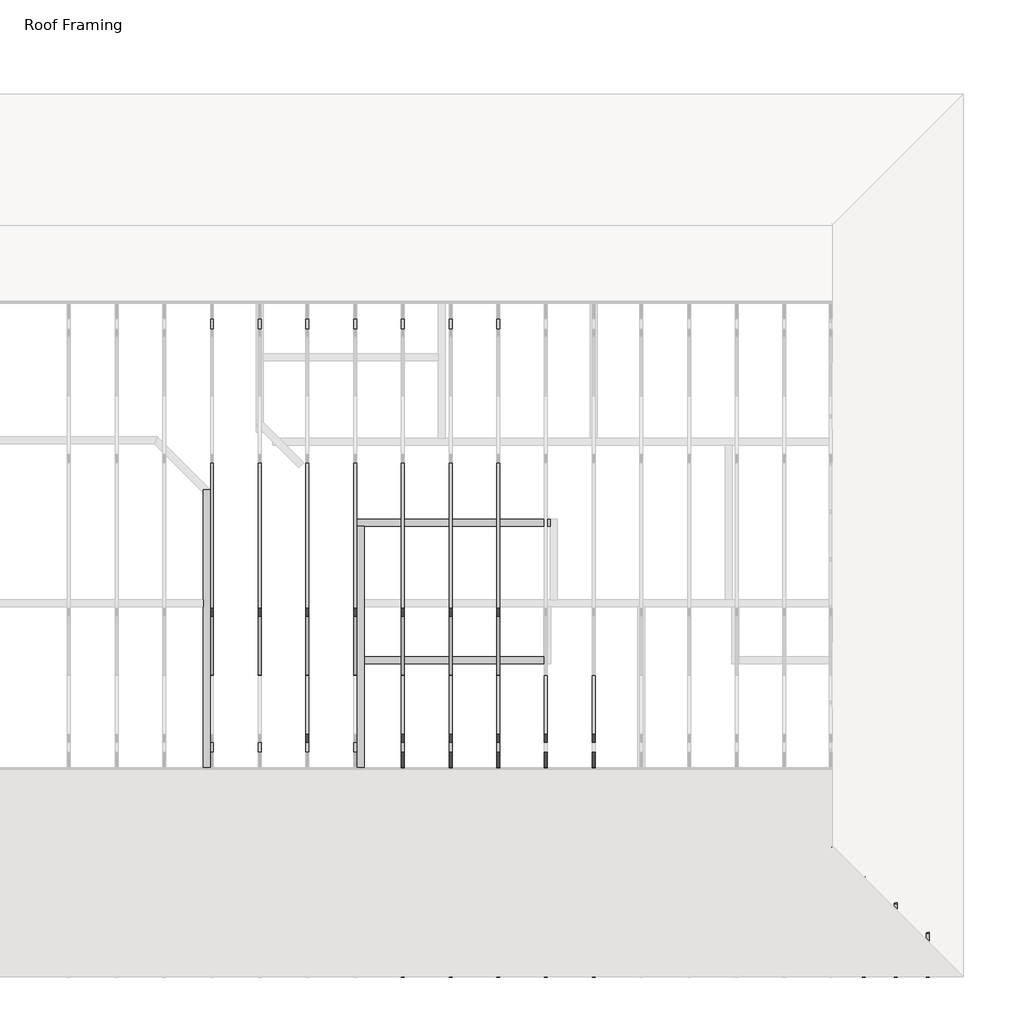
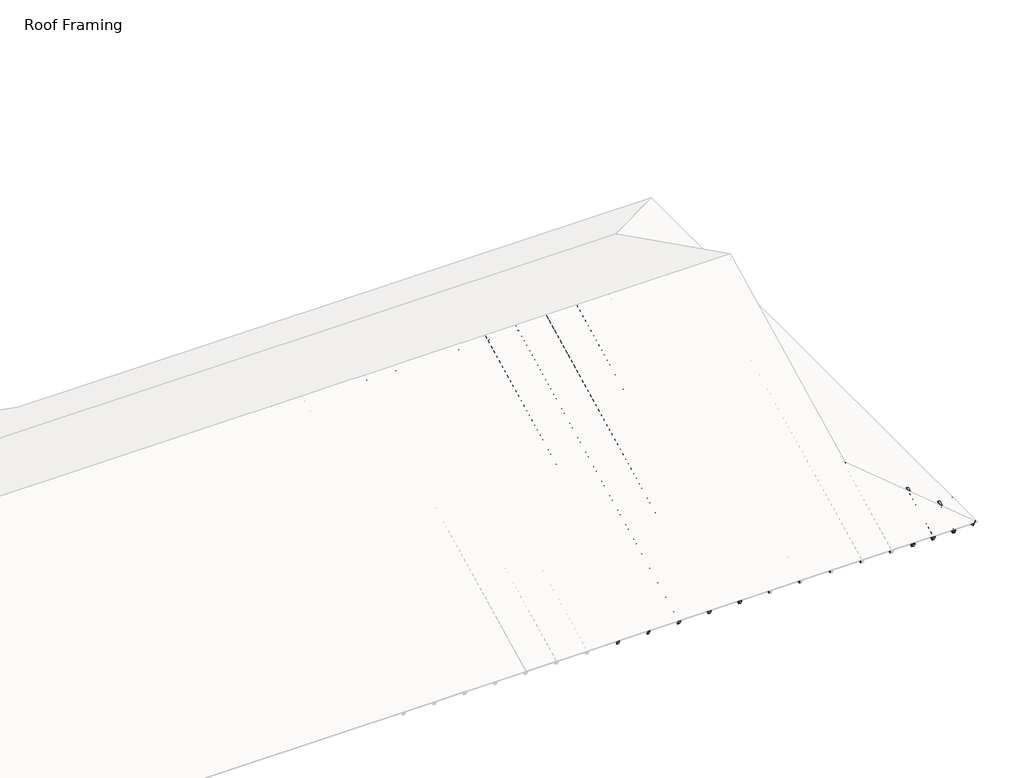
# One storey, part 3 of 7: 48 beams, 13 members.
"""IFC4 building model written with IfcOpenShell, lengths in millimetres."""

import ifcopenshell
import ifcopenshell.guid

model = None  # the IFC model being written
_history = None  # IfcOwnerHistory: only IFC2X3 demands one
_inside = {}  # id of a spatial element -> (the spatial element, [elements in it])
_under = {}  # id of a project, library or spatial element -> (it, [spatial elements below it])
_declared = {}  # id of a project -> (the project, [libraries it declares])
_typed = {}  # id of a type object -> (the type object, [elements of that type])
_made_of = {}  # id of a material, layer set ... -> (it, [elements and type objects made of it])


def new_model(schema):
    """Start an empty IFC model of exactly this schema.

    Asked for "IFC4X3", IfcOpenShell would pick the latest addendum, in which some entities
    have other attributes; the version numbers below select the first issue.
    IFC2X3 requires an IfcOwnerHistory on every rooted entity: one is made here for all.
    """
    global model, _history
    if schema == "IFC4X3":
        model = ifcopenshell.file(schema_version=(4, 3, 0, 0))
    else:
        model = ifcopenshell.file(schema=schema)
    _inside.clear()
    _under.clear()
    _declared.clear()
    _typed.clear()
    _made_of.clear()
    _history = None
    if model.schema == "IFC2X3":
        org = make("IfcOrganization", Name="unknown")
        user = make(
            "IfcPersonAndOrganization",
            ThePerson=make("IfcPerson", FamilyName="unknown"),
            TheOrganization=org,
        )
        app = make(
            "IfcApplication",
            ApplicationDeveloper=org,
            Version="unknown",
            ApplicationFullName="unknown",
            ApplicationIdentifier="unknown",
        )
        _history = make(
            "IfcOwnerHistory",
            OwningUser=user,
            OwningApplication=app,
            ChangeAction="ADDED",
            CreationDate=0,
        )
    return model


def make(cls, **values):
    """One entity of the class cls with the attributes given. An attribute that is None is left unset."""
    return model.create_entity(
        cls, **{name: value for name, value in values.items() if value is not None}
    )


def rooted(cls, **values):
    """An entity with a GlobalId (a new one), such as an element, a storey or a relation."""
    return make(cls, GlobalId=ifcopenshell.guid.new(), OwnerHistory=_history, **values)


def si_unit(unit_type, name, prefix=None):
    """IfcSIUnit, for example si_unit("LENGTHUNIT", "METRE", prefix="MILLI")."""
    return make("IfcSIUnit", UnitType=unit_type, Prefix=prefix, Name=name)


def assignment(units):
    """IfcUnitAssignment: the units of a project."""
    return None if units is None else make("IfcUnitAssignment", Units=units)


def point(xyz):
    """IfcCartesianPoint."""
    return None if xyz is None else make("IfcCartesianPoint", Coordinates=xyz)


def direction(xyz):
    """IfcDirection."""
    return None if xyz is None else make("IfcDirection", DirectionRatios=xyz)


def frame(location, z_axis=None, x_axis=None):
    """IfcAxis2Placement3D, a coordinate frame: its origin and axes. An axis left out is left unset."""
    return make(
        "IfcAxis2Placement3D",
        Location=point(location),
        Axis=direction(z_axis),
        RefDirection=direction(x_axis),
    )


def origin():
    """The frame at (0, 0, 0) with its axes left unset."""
    return frame((0.0, 0.0, 0.0))


def place(relative_to, where):
    """IfcLocalPlacement: puts the frame where relative to a parent placement (None: the world)."""
    return make(
        "IfcLocalPlacement", PlacementRelTo=relative_to, RelativePlacement=where
    )


def context(
    kind, dimensions, precision=None, world=None, true_north=None, identifier=None
):
    """IfcGeometricRepresentationContext, for example the 3D "Model" context."""
    return make(
        "IfcGeometricRepresentationContext",
        ContextIdentifier=identifier,
        ContextType=kind,
        CoordinateSpaceDimension=dimensions,
        Precision=precision,
        WorldCoordinateSystem=world,
        TrueNorth=true_north,
    )


def project(units=None, contexts=None):
    """IfcProject with its units and contexts."""
    return rooted(
        "IfcProject",
        Name="project",
        RepresentationContexts=contexts,
        UnitsInContext=assignment(units),
    )


def spatial(cls, under=None, at=None, **own):
    """A site, building, storey or space (cls), placed at a placement, below another one or the project."""
    s = rooted(cls, ObjectPlacement=at, **own)
    if under is not None:
        _under.setdefault(under.id(), (under, []))[1].append(s)
    return s


def polyline(points):
    """IfcPolyline through the points."""
    return make("IfcPolyline", Points=[point(p) for p in points])


def outline(outer, holes=None, kind="AREA"):
    """IfcArbitraryClosedProfileDef: a profile drawn as a closed curve; with holes, ...WithVoids."""
    if holes is None:
        return make("IfcArbitraryClosedProfileDef", ProfileType=kind, OuterCurve=outer)
    return make(
        "IfcArbitraryProfileDefWithVoids",
        ProfileType=kind,
        OuterCurve=outer,
        InnerCurves=holes,
    )


def extrude(swept, where, along, depth):
    """IfcExtrudedAreaSolid: the profile swept, set in the frame where, extruded along a direction by depth."""
    return make(
        "IfcExtrudedAreaSolid",
        SweptArea=swept,
        Position=where,
        ExtrudedDirection=direction(along),
        Depth=depth,
    )


def faces_of(points, faces, orient=None, outer=None):
    """IfcFace entities. A face is a list of loops; a loop is a list of indices into points, from 0.

    orient and outer hold one flag for each loop. By default every Orientation is true, the
    first loop of a face is its IfcFaceOuterBound and the others are IfcFaceBound.
    """
    made = []
    for i, loops in enumerate(faces):
        bounds = []
        for j, loop in enumerate(loops):
            is_outer = j == 0 if outer is None else outer[i][j]
            bounds.append(
                make(
                    "IfcFaceOuterBound" if is_outer else "IfcFaceBound",
                    Bound=make("IfcPolyLoop", Polygon=[points[k] for k in loop]),
                    Orientation=True if orient is None else orient[i][j],
                )
            )
        made.append(make("IfcFace", Bounds=bounds))
    return made


def faceted_brep(points, faces, orient=None, outer=None, voids=None):
    """IfcFacetedBrep: a solid bounded by flat faces; with voids (closed shells), ...WithVoids."""
    shared = [point(p) for p in points]
    hull = make("IfcClosedShell", CfsFaces=faces_of(shared, faces, orient, outer))
    if voids is None:
        return make("IfcFacetedBrep", Outer=hull)
    return make(
        "IfcFacetedBrepWithVoids",
        Outer=hull,
        Voids=[
            make(cls, CfsFaces=faces_of(shared, fs, o, b)) for cls, fs, o, b in voids
        ],
    )


def shape(context_of_items, identifier, shape_type, items):
    """IfcShapeRepresentation: the items that make up one representation, for example the "Body"."""
    return make(
        "IfcShapeRepresentation",
        ContextOfItems=context_of_items,
        RepresentationIdentifier=identifier,
        RepresentationType=shape_type,
        Items=items,
    )


def source(mapping_origin, context_of_items, identifier, shape_type, items):
    """IfcRepresentationMap: a shape defined once, which mapped items show again and again."""
    return make(
        "IfcRepresentationMap",
        MappingOrigin=mapping_origin,
        MappedRepresentation=shape(context_of_items, identifier, shape_type, items),
    )


def transform(
    local_origin,
    x_axis=None,
    y_axis=None,
    z_axis=None,
    scale=None,
    scale2=None,
    scale3=None,
    uniform=True,
):
    """IfcCartesianTransformationOperator3D, or its non-uniform kind. x_axis, y_axis, z_axis: its Axis1, 2, 3."""
    if uniform:
        return make(
            "IfcCartesianTransformationOperator3D",
            Axis1=direction(x_axis),
            Axis2=direction(y_axis),
            LocalOrigin=point(local_origin),
            Scale=scale,
            Axis3=direction(z_axis),
        )
    return make(
        "IfcCartesianTransformationOperator3DnonUniform",
        Axis1=direction(x_axis),
        Axis2=direction(y_axis),
        LocalOrigin=point(local_origin),
        Scale=scale,
        Axis3=direction(z_axis),
        Scale2=scale2,
        Scale3=scale3,
    )


def mapped(mapping_source, mapping_target):
    """IfcMappedItem: shows the shape of a source again, moved by a transform."""
    return make(
        "IfcMappedItem", MappingSource=mapping_source, MappingTarget=mapping_target
    )


def made_of(thing, what):
    """Note that an element or type object is made of a material, layer set ...; save() writes the relation."""
    if what is not None:
        _made_of.setdefault(what.id(), (what, []))[1].append(thing)
    return thing


def element(
    cls,
    number,
    at=None,
    inside=None,
    cuts=None,
    type_object=None,
    material=None,
    context=None,
    identifier="Body",
    shape_type=None,
    held_by="IfcProductDefinitionShape",
    body=None,
    shapes=None,
    **own,
):
    """One element of the class cls, such as IfcWall. Its Tag is "e" and its number.

    at: its placement. inside: the storey or other place that contains it. cuts: it is an
    opening in that element (IfcRelVoidsElement). A single representation is given by context,
    identifier, shape_type and body (its items); several are given by shapes. held_by: the class
    of the entity that holds the representations. save() writes the other relations.
    """
    e = rooted(cls, Tag="e%d" % number, ObjectPlacement=at, **own)
    if body is not None:
        shapes = [shape(context, identifier, shape_type, body)]
    if shapes is not None:
        e.Representation = make(held_by, Representations=shapes)
    if inside is not None:
        _inside.setdefault(inside.id(), (inside, []))[1].append(e)
    if cuts is not None:
        rooted(
            "IfcRelVoidsElement", RelatingBuildingElement=cuts, RelatedOpeningElement=e
        )
    if type_object is not None:
        _typed.setdefault(type_object.id(), (type_object, []))[1].append(e)
    return made_of(e, material)


def aggregate(whole, parts):
    """IfcRelAggregates: a whole, such as a stair, and the parts it consists of."""
    return rooted("IfcRelAggregates", RelatingObject=whole, RelatedObjects=parts)


def save(model, path):
    """Write the relations noted so far, then the file.

    IfcRelAggregates (storeys below a building ...), IfcRelContainedInSpatialStructure (elements
    in a storey), IfcRelDefinesByType, IfcRelAssociatesMaterial and IfcRelDeclares: one each for
    every whole, place, type object, material and project.
    """
    for whole, parts in _under.values():
        aggregate(whole, parts)
    for where, things in _inside.values():
        rooted(
            "IfcRelContainedInSpatialStructure",
            RelatedElements=things,
            RelatingStructure=where,
        )
    for kind, things in _typed.values():
        rooted("IfcRelDefinesByType", RelatedObjects=things, RelatingType=kind)
    for what, things in _made_of.values():
        rooted("IfcRelAssociatesMaterial", RelatedObjects=things, RelatingMaterial=what)
    for by, libraries in _declared.values():
        rooted("IfcRelDeclares", RelatingContext=by, RelatedDefinitions=libraries)
    model.write(path)


def dimension_lumber_a2ec78f1(model_context):
    return source(origin(), model_context, "Body", "SweptSolid", [
        extrude(outline(polyline([(1250.4988621, -19.05), (-1215.9128821, -19.05), (-1215.9128821, 19.05), (1250.4988621, 19.05), (1250.4988621, -19.05)])), frame((0.0, 0.0, -44.45), z_axis=(0.0, 0.0, 1.0), x_axis=(1.0, 0.0, 0.0)), (0.0, 0.0, 1.0), 88.9),
    ])


def dimension_lumber_a36e28ec(model_context):
    return source(origin(), model_context, "Body", "SweptSolid", [
        extrude(outline(polyline([(3639.34375, 44.45), (3639.34375, -44.45), (-3550.44375, -44.45), (-3550.44375, 44.45), (3639.34375, 44.45)])), frame((0.0, 0.0, -19.05), z_axis=(0.0, 0.0, 1.0), x_axis=(1.0, 0.0, 0.0)), (0.0, 0.0, 1.0), 38.1),
    ])


def dimension_lumber_e4f6bc88(model_context):
    return source(origin(), model_context, "Body", "SweptSolid", [
        extrude(outline(polyline([(5029.99375, 44.45), (5029.99375, -44.45), (3696.49375, -44.45), (3696.49375, 44.45), (5029.99375, 44.45)])), frame((0.0, 0.0, -19.05), z_axis=(0.0, 0.0, 1.0), x_axis=(1.0, 0.0, 0.0)), (0.0, 0.0, 1.0), 38.1),
    ])


def dimension_lumber_71d4a028(model_context):
    return source(origin(), model_context, "Body", "SweptSolid", [
        extrude(outline(polyline([(5096.66875, -44.45), (3674.26875, -44.45), (3674.26875, 44.45), (5096.66875, 44.45), (5096.66875, -44.45)])), frame((0.0, 0.0, -19.05), z_axis=(0.0, 0.0, 1.0), x_axis=(1.0, 0.0, 0.0)), (0.0, 0.0, 1.0), 38.1),
    ])


def dimension_lumber_ec547c4e(model_context):
    return source(origin(), model_context, "Body", "SweptSolid", [
        extrude(outline(polyline([(1866.9, 44.45), (1866.9, -44.45), (-1809.75, -44.45), (-1809.75, 44.45), (1866.9, 44.45)])), frame((0.0, 0.0, -19.05), z_axis=(0.0, 0.0, 1.0), x_axis=(1.0, 0.0, 0.0)), (0.0, 0.0, 1.0), 38.1),
    ])


def dimension_lumber_8a2991dc(model_context):
    return source(origin(), model_context, "Body", "SweptSolid", [
        extrude(outline(polyline([(1279.525, 44.45), (1279.525, -44.45), (-1190.625, -44.45), (-1190.625, 44.45), (1279.525, 44.45)])), frame((0.0, 0.0, -19.05), z_axis=(0.0, 0.0, 1.0), x_axis=(1.0, 0.0, 0.0)), (0.0, 0.0, 1.0), 38.1),
    ])


def dimension_lumber_bb8f2985(model_context):
    return source(origin(), model_context, "Body", "SweptSolid", [
        extrude(outline(polyline([(1149.3500003, 44.45), (1149.3500003, -44.45), (-1149.3500003, -44.45), (-1149.3500003, 44.45), (1149.3500003, 44.45)])), frame((0.0, 0.0, -19.05), z_axis=(0.0, 0.0, 1.0), x_axis=(1.0, 0.0, 0.0)), (0.0, 0.0, 1.0), 38.1),
    ])


def dimension_lumber_e331b447(model_context):
    return source(origin(), model_context, "Body", "SweptSolid", [
        extrude(outline(polyline([(1838.325, 44.45), (1838.325, -44.45), (-1838.325, -44.45), (-1838.325, 44.45), (1838.325, 44.45)])), frame((0.0, 0.0, -19.05), z_axis=(0.0, 0.0, 1.0), x_axis=(1.0, 0.0, 0.0)), (0.0, 0.0, 1.0), 38.1),
    ])


def dimension_lumber_3e8a9e7d(model_context):
    return source(origin(), model_context, "Body", "SweptSolid", [
        extrude(outline(polyline([(1158.8750006, 44.45), (1158.8750006, -44.45), (-1139.825, -44.45), (-1139.825, 44.45), (1158.8750006, 44.45)])), frame((0.0, 0.0, -19.05), z_axis=(0.0, 0.0, 1.0), x_axis=(1.0, 0.0, 0.0)), (0.0, 0.0, 1.0), 38.1),
    ])


model = new_model("IFC4")

# Units and contexts
model_context = context("Model", 3, world=origin())
ifc_project = project(units=[si_unit("LENGTHUNIT", "METRE", prefix="MILLI")], contexts=[model_context])

# Site, building, storey
site = spatial("IfcSite", under=ifc_project)
building = spatial("IfcBuilding", under=site)
storey = spatial("IfcBuildingStorey", under=building, Name="Roof Framing", Elevation=2768.6)

# Beams
placement = place(None, origin())
element("IfcBeam", 1, ObjectType="Dimension Lumber : Roof Lumbers", at=placement, inside=storey, context=model_context, shape_type="SweptSolid", body=[
    extrude(outline(polyline([(0.0, -38.1), (0.0, 0.0), (1874.2721787, 0.0), (1874.2721787, -38.1), (0.0, -38.1)])), frame((13672.6274862, -4054.1040947, 2554.840297), z_axis=(0.4472135954999341, 0.0, 0.8944271909999277), x_axis=(-0.8944271909999277, 0.0, 0.4472135954999341)), (0.0, 0.0, 1.0), 88.9),
    extrude(outline(polyline([(2554.840297, 13672.6274862), (2558.1548743, 13674.2847749), (2653.4048743, 13674.2847749), (3472.5548743, 12035.9847749), (3393.040297, 11996.2274862), (2554.840297, 13672.6274862)])), frame((0.0, -4054.1040947, 0.0), z_axis=(0.0, 1.0, 0.0), x_axis=(0.0, 0.0, 1.0)), (0.0, 0.0, 1.0), 38.1),
    extrude(outline(polyline([(2554.840297, 13672.6274862), (2558.1548743, 13674.2847749), (2653.4048743, 13674.2847749), (3472.5548743, 12035.9847749), (3373.1616527, 12035.9847749), (2554.840297, 13672.6274862)])), frame((0.0, -4054.1040947, 0.0), z_axis=(0.0, 1.0, 0.0), x_axis=(0.0, 0.0, 1.0)), (0.0, 0.0, 1.0), 38.1),
])
element("IfcBeam", 2, ObjectType="Dimension Lumber : Roof Lumbers", at=placement, inside=storey, context=model_context, shape_type="SweptSolid", body=[
    extrude(outline(polyline([(12035.9847749, -4625.6040947), (13244.0722749, -4625.6040947), (13244.0722749, -4663.7040947), (12035.9847749, -4663.7040947), (12035.9847749, -4625.6040947)])), frame((0.0, 0.0, 2768.6), z_axis=(0.0, 0.0, 1.0), x_axis=(1.0, 0.0, 0.0)), (0.0, 0.0, 1.0), 88.9),
    extrude(outline(polyline([(2768.6, 12035.9847749), (2768.6, 13244.0722749), (2769.1179027, 13244.0722749), (2857.5, 13067.3080803), (2857.5, 12035.9847749), (2768.6, 12035.9847749)])), frame((0.0, -4663.7040947, 0.0), z_axis=(0.0, 1.0, 0.0), x_axis=(0.0, 0.0, 1.0)), (0.0, 0.0, 1.0), 38.1),
])
element("IfcBeam", 3, ObjectType="Dimension Lumber : Roof Lumbers", at=placement, inside=storey, context=model_context, shape_type="SweptSolid", body=[
    extrude(outline(polyline([(0.0, 38.1), (1874.2721787, 38.1), (1874.2721787, 0.0), (0.0, 0.0), (0.0, 38.1)])), frame((13672.6274862, -4016.0040947, 2554.840297), z_axis=(0.4472135954999341, 0.0, 0.8944271909999277), x_axis=(-0.8944271909999277, 0.0, 0.4472135954999341)), (0.0, 0.0, 1.0), 88.9),
    extrude(outline(polyline([(2653.4048743, 13674.2847749), (3472.5548743, 12035.9847749), (3393.040297, 11996.2274862), (2554.840297, 13672.6274862), (2558.1548743, 13674.2847749), (2653.4048743, 13674.2847749)])), frame((0.0, -4054.1040947, 0.0), z_axis=(0.0, 1.0, 0.0), x_axis=(0.0, 0.0, 1.0)), (0.0, 0.0, 1.0), 38.1),
    extrude(outline(polyline([(2653.4048743, 13674.2847749), (3472.5548743, 12035.9847749), (3373.1616527, 12035.9847749), (2554.840297, 13672.6274862), (2558.1548743, 13674.2847749), (2653.4048743, 13674.2847749)])), frame((0.0, -4054.1040947, 0.0), z_axis=(0.0, 1.0, 0.0), x_axis=(0.0, 0.0, 1.0)), (0.0, 0.0, 1.0), 38.1),
])
element("IfcBeam", 4, ObjectType="Dimension Lumber : Roof Lumbers", at=placement, inside=storey, context=model_context, shape_type="SweptSolid", body=[
    extrude(outline(polyline([(0.0, 38.1), (1877.070187, 38.1), (1877.070187, 0.0), (0.0, 0.0), (0.0, 38.1)])), frame((13672.6274862, -4625.6040947, 2554.840297), z_axis=(0.4472135954999341, 0.0, 0.8944271909999277), x_axis=(-0.8944271909999277, 0.0, 0.4472135954999341)), (0.0, 0.0, 1.0), 88.9),
    extrude(outline(polyline([(2653.4048743, 13674.2847749), (3473.8061816, 12033.4821602), (3394.2916044, 11993.7248716), (2554.840297, 13672.6274862), (2558.1548743, 13674.2847749), (2653.4048743, 13674.2847749)])), frame((0.0, -4663.7040947, 0.0), z_axis=(0.0, 1.0, 0.0), x_axis=(0.0, 0.0, 1.0)), (0.0, 0.0, 1.0), 38.1),
    extrude(outline(polyline([(2653.4048743, 13674.2847749), (3472.5548743, 12035.9847749), (3373.1616527, 12035.9847749), (2554.840297, 13672.6274862), (2558.1548743, 13674.2847749), (2653.4048743, 13674.2847749)])), frame((0.0, -4663.7040947, 0.0), z_axis=(0.0, 1.0, 0.0), x_axis=(0.0, 0.0, 1.0)), (0.0, 0.0, 1.0), 38.1),
])
element("IfcBeam", 5, ObjectType="Dimension Lumber : Roof Lumbers", at=placement, inside=storey, context=model_context, shape_type="SweptSolid", body=[
    extrude(outline(polyline([(12035.9847749, -4016.0040947), (13244.0722749, -4016.0040947), (13244.0722749, -4054.1040947), (12035.9847749, -4054.1040947), (12035.9847749, -4016.0040947)])), frame((0.0, 0.0, 2768.6), z_axis=(0.0, 0.0, 1.0), x_axis=(1.0, 0.0, 0.0)), (0.0, 0.0, 1.0), 88.9),
    extrude(outline(polyline([(2768.6, 12035.9847749), (2768.6, 13244.0722749), (2769.1179027, 13244.0722749), (2857.5, 13067.3080803), (2857.5, 12035.9847749), (2768.6, 12035.9847749)])), frame((0.0, -4054.1040947, 0.0), z_axis=(0.0, 1.0, 0.0), x_axis=(0.0, 0.0, 1.0)), (0.0, 0.0, 1.0), 38.1),
])
element("IfcBeam", 6, ObjectType="Dimension Lumber : Top Supporting Lumbers", at=placement, inside=storey, context=model_context, shape_type="SweptSolid", body=[
    extrude(outline(polyline([(3996.8847749, -98.0540947), (4085.7847749, -98.0540947), (4085.7847749, -4238.2540947), (3996.8847749, -4238.2540947), (3996.8847749, -98.0540947)])), frame((0.0, 0.0, 2692.4), z_axis=(0.0, 0.0, 1.0), x_axis=(1.0, 0.0, 0.0)), (0.0, 0.0, 1.0), 38.1),
    extrude(outline(polyline([(4085.7847749, -98.0540947), (4085.7847749, -4238.2540947), (3996.8847749, -4238.2540947), (3996.8847749, -134.8776804), (4085.7847749, -98.0540947)])), frame((0.0, 0.0, 2692.4), z_axis=(0.0, 0.0, 1.0), x_axis=(1.0, 0.0, 0.0)), (0.0, 0.0, 1.0), 38.1),
])
element("IfcBeam", 7, ObjectType="Dimension Lumber : Roof Lumbers", at=placement, inside=storey, context=model_context, shape_type="Brep", body=[
    faceted_brep([(12461.4347749, -5041.9472419, 3273.9083007), (12461.4347749, -5002.1899532, 3194.3937234), (12423.3347749, -5002.1899532, 3194.3937234), (12423.3347749, -5041.9472419, 3273.9083007), (12461.4347749, -6329.0380921, 2630.3628756), (12423.3347749, -6329.0380921, 2630.3628756), (12423.3347749, -6289.2808035, 2550.8482983), (12461.4347749, -6289.2808035, 2550.8482983)], [[[0, 1, 2, 3]], [[4, 5, 6, 7]], [[3, 5, 4, 0]], [[2, 6, 5, 3]], [[1, 7, 6, 2]], [[0, 4, 7, 1]]]),
    faceted_brep([(12461.4347749, -6329.0380921, 2630.3628756), (12423.3347749, -6329.0380921, 2630.3628756), (12423.3347749, -6289.2808035, 2550.8482983), (12461.4347749, -6289.2808035, 2550.8482983), (12423.3347749, -5058.9448631, 3265.4094901), (12461.4347749, -5097.0448631, 3246.3594901), (12423.3347749, -5058.9448631, 3166.0162685), (12461.4347749, -5097.0448631, 3146.9662685)], [[[0, 1, 2, 3]], [[4, 1, 0, 5]], [[6, 2, 1, 4]], [[7, 3, 2, 6]], [[5, 0, 3, 7]], [[4, 5, 7, 6]]]),
    faceted_brep([(12461.4347749, -6329.0380921, 2630.3628756), (12423.3347749, -6329.0380921, 2630.3628756), (12423.3347749, -6296.1597793, 2564.60625), (12461.4347749, -6296.1597793, 2564.60625), (12423.3347749, -5058.9448631, 3265.4094901), (12461.4347749, -5097.0448631, 3246.3594901), (12423.3347749, -5058.9448631, 3166.0162685), (12423.3347749, -6261.7649001, 2564.60625), (12461.4347749, -6261.7649001, 2564.60625), (12461.4347749, -5097.0448631, 3146.9662685)], [[[0, 1, 2, 3]], [[4, 1, 0, 5]], [[6, 7, 2, 1, 4]], [[5, 0, 3, 8, 9]], [[4, 5, 9, 6]], [[9, 8, 7, 6]], [[3, 2, 7, 8]]]),
    faceted_brep([(12423.3347749, -5058.9448631, 3166.0162685), (12423.3347749, -6261.7649001, 2564.60625), (12423.3347749, -6282.9540947, 2564.60625), (12423.3347749, -6282.9540947, 2653.4048743), (12423.3347749, -5058.9448631, 3265.4094901), (12461.4347749, -6282.9540947, 2653.4048743), (12461.4347749, -5097.0448631, 3246.3594901), (12461.4347749, -6282.9540947, 2564.60625), (12461.4347749, -6261.7649001, 2564.60625), (12461.4347749, -5097.0448631, 3146.9662685)], [[[0, 1, 2, 3, 4]], [[4, 3, 5, 6]], [[6, 5, 7, 8, 9]], [[4, 6, 9, 0]], [[9, 8, 1, 0]], [[2, 1, 8, 7]], [[5, 3, 2, 7]]]),
])
element("IfcBeam", 8, ObjectType="Dimension Lumber : Roof Lumbers", at=placement, inside=storey, context=model_context, shape_type="Brep", body=[
    faceted_brep([(12867.8347749, -5385.152618, 3102.3056127), (12867.8347749, -5345.3953294, 3022.7910354), (12829.7347749, -5345.3953294, 3022.7910354), (12829.7347749, -5385.152618, 3102.3056127), (12867.8347749, -6329.0380921, 2630.3628756), (12829.7347749, -6329.0380921, 2630.3628756), (12829.7347749, -6289.2808035, 2550.8482983), (12867.8347749, -6289.2808035, 2550.8482983)], [[[0, 1, 2, 3]], [[4, 5, 6, 7]], [[3, 5, 4, 0]], [[2, 6, 5, 3]], [[1, 7, 6, 2]], [[0, 4, 7, 1]]]),
    faceted_brep([(12867.8347749, -6329.0380921, 2630.3628756), (12829.7347749, -6329.0380921, 2630.3628756), (12829.7347749, -6289.2808035, 2550.8482983), (12867.8347749, -6289.2808035, 2550.8482983), (12829.7347749, -5465.3448631, 3062.2094901), (12867.8347749, -5503.4448631, 3043.1594901), (12829.7347749, -5465.3448631, 2962.8162685), (12867.8347749, -5503.4448631, 2943.7662685)], [[[0, 1, 2, 3]], [[4, 1, 0, 5]], [[6, 2, 1, 4]], [[7, 3, 2, 6]], [[5, 0, 3, 7]], [[4, 5, 7, 6]]]),
    faceted_brep([(12867.8347749, -6329.0380921, 2630.3628756), (12829.7347749, -6329.0380921, 2630.3628756), (12829.7347749, -6296.1597793, 2564.60625), (12867.8347749, -6296.1597793, 2564.60625), (12829.7347749, -5465.3448631, 3062.2094901), (12867.8347749, -5503.4448631, 3043.1594901), (12829.7347749, -5465.3448631, 2962.8162685), (12829.7347749, -6261.7649001, 2564.60625), (12867.8347749, -6261.7649001, 2564.60625), (12867.8347749, -5503.4448631, 2943.7662685)], [[[0, 1, 2, 3]], [[4, 1, 0, 5]], [[6, 7, 2, 1, 4]], [[5, 0, 3, 8, 9]], [[4, 5, 9, 6]], [[9, 8, 7, 6]], [[3, 2, 7, 8]]]),
    faceted_brep([(12829.7347749, -5465.3448631, 2962.8162685), (12829.7347749, -6261.7649001, 2564.60625), (12829.7347749, -6282.9540947, 2564.60625), (12829.7347749, -6282.9540947, 2653.4048743), (12829.7347749, -5465.3448631, 3062.2094901), (12867.8347749, -6282.9540947, 2653.4048743), (12867.8347749, -5503.4448631, 3043.1594901), (12867.8347749, -6282.9540947, 2564.60625), (12867.8347749, -6261.7649001, 2564.60625), (12867.8347749, -5503.4448631, 2943.7662685)], [[[0, 1, 2, 3, 4]], [[4, 3, 5, 6]], [[6, 5, 7, 8, 9]], [[4, 6, 9, 0]], [[9, 8, 1, 0]], [[2, 1, 8, 7]], [[5, 3, 2, 7]]]),
])
element("IfcBeam", 9, ObjectType="Dimension Lumber : Roof Lumbers", at=placement, inside=storey, context=model_context, shape_type="Brep", body=[
    faceted_brep([(13274.2347749, -5771.3662791, 2909.1987821), (13274.2347749, -5731.6089904, 2829.6842048), (13236.1347749, -5731.6089904, 2829.6842048), (13236.1347749, -5771.3662791, 2909.1987821), (13274.2347749, -6329.0380921, 2630.3628756), (13236.1347749, -6329.0380921, 2630.3628756), (13236.1347749, -6289.2808035, 2550.8482983), (13274.2347749, -6289.2808035, 2550.8482983)], [[[0, 1, 2, 3]], [[4, 5, 6, 7]], [[3, 5, 4, 0]], [[2, 6, 5, 3]], [[1, 7, 6, 2]], [[0, 4, 7, 1]]]),
    faceted_brep([(13274.2347749, -6329.0380921, 2630.3628756), (13236.1347749, -6329.0380921, 2630.3628756), (13236.1347749, -6289.2808035, 2550.8482983), (13274.2347749, -6289.2808035, 2550.8482983), (13236.1347749, -5871.7448631, 2859.0094901), (13274.2347749, -5909.8448631, 2839.9594901), (13236.1347749, -5871.7448631, 2759.6162685), (13274.2347749, -5909.8448631, 2740.5662685)], [[[0, 1, 2, 3]], [[4, 1, 0, 5]], [[6, 2, 1, 4]], [[7, 3, 2, 6]], [[5, 0, 3, 7]], [[4, 5, 7, 6]]]),
    faceted_brep([(13274.2347749, -6329.0380921, 2630.3628756), (13236.1347749, -6329.0380921, 2630.3628756), (13236.1347749, -6296.1597793, 2564.60625), (13274.2347749, -6296.1597793, 2564.60625), (13236.1347749, -5871.7448631, 2859.0094901), (13274.2347749, -5909.8448631, 2839.9594901), (13236.1347749, -5871.7448631, 2759.6162685), (13236.1347749, -6261.7649001, 2564.60625), (13274.2347749, -6261.7649001, 2564.60625), (13274.2347749, -5909.8448631, 2740.5662685)], [[[0, 1, 2, 3]], [[4, 1, 0, 5]], [[6, 7, 2, 1, 4]], [[5, 0, 3, 8, 9]], [[4, 5, 9, 6]], [[9, 8, 7, 6]], [[3, 2, 7, 8]]]),
    faceted_brep([(13236.1347749, -5871.7448631, 2759.6162685), (13236.1347749, -6261.7649001, 2564.60625), (13236.1347749, -6282.9540947, 2564.60625), (13236.1347749, -6282.9540947, 2653.4048743), (13236.1347749, -5871.7448631, 2859.0094901), (13274.2347749, -6282.9540947, 2653.4048743), (13274.2347749, -5909.8448631, 2839.9594901), (13274.2347749, -6282.9540947, 2564.60625), (13274.2347749, -6261.7649001, 2564.60625), (13274.2347749, -5909.8448631, 2740.5662685)], [[[0, 1, 2, 3, 4]], [[4, 3, 5, 6]], [[6, 5, 7, 8, 9]], [[4, 6, 9, 0]], [[9, 8, 1, 0]], [[2, 1, 8, 7]], [[5, 3, 2, 7]]]),
])
dimension_lumber_shape = dimension_lumber_a2ec78f1(model_context)
element("IfcBeam", 10, ObjectType="Dimension Lumber : Roof Lumbers", at=placement, inside=storey, context=model_context, shape_type="MappedRepresentation", body=[
    mapped(dimension_lumber_shape, transform((12862.2111001, -5470.8804199, 3005.560175), x_axis=(-0.6666666666666689, 0.666666666666668, 0.33333333333332643), y_axis=(-0.7071067811865471, -0.7071067811865481, 0.0), z_axis=(0.23570226039551126, -0.23570226039551093, 0.9428090415820658))),
])
dimension_lumber_2_shape = dimension_lumber_a36e28ec(model_context)
element("IfcBeam", 11, ObjectType="Dimension Lumber : Top Supporting Lumbers", at=placement, inside=storey, context=model_context, shape_type="MappedRepresentation", body=[
    mapped(dimension_lumber_2_shape, transform((9604.7285249, -5705.1040947, 2711.45), x_axis=(-1.0, 0.0, 0.0), y_axis=(0.0, -1.0, 0.0), z_axis=(0.0, 0.0, 1.0))),
])
dimension_lumber_3_shape = dimension_lumber_e4f6bc88(model_context)
element("IfcBeam", 12, ObjectType="Dimension Lumber : Top Supporting Lumbers", at=placement, inside=storey, context=model_context, shape_type="MappedRepresentation", body=[
    mapped(dimension_lumber_3_shape, transform((6009.8347749, -630.6603447, 2749.55), x_axis=(0.0, -1.0, 0.0), y_axis=(1.0, 0.0, 0.0), z_axis=(0.0, 0.0, 1.0))),
])
element("IfcBeam", 13, ObjectType="Dimension Lumber : Top Supporting Lumbers", at=placement, inside=storey, context=model_context, shape_type="MappedRepresentation", body=[
    mapped(dimension_lumber_3_shape, transform((6009.8347749, -630.6603447, 2711.45), x_axis=(0.0, -1.0, 0.0), y_axis=(1.0, 0.0, 0.0), z_axis=(0.0, 0.0, 1.0))),
])
dimension_lumber_4_shape = dimension_lumber_71d4a028(model_context)
element("IfcBeam", 14, ObjectType="Dimension Lumber : Top Supporting Lumbers", at=placement, inside=storey, context=model_context, shape_type="MappedRepresentation", body=[
    mapped(dimension_lumber_4_shape, transform((4041.3347749, -652.8853447, 2749.55), x_axis=(0.0, -1.0, 0.0), y_axis=(1.0, 0.0, 0.0), z_axis=(0.0, 0.0, 1.0))),
])
element("IfcBeam", 15, ObjectType="Dimension Lumber : Top Supporting Lumbers", at=placement, inside=storey, context=model_context, shape_type="MappedRepresentation", body=[
    mapped(dimension_lumber_4_shape, transform((4041.3347749, -652.8853447, 2711.45), x_axis=(0.0, -1.0, 0.0), y_axis=(1.0, 0.0, 0.0), z_axis=(0.0, 0.0, 1.0))),
])
dimension_lumber_5_shape = dimension_lumber_ec547c4e(model_context)
element("IfcBeam", 16, ObjectType="Dimension Lumber : Top Supporting Lumbers", at=placement, inside=storey, context=model_context, shape_type="MappedRepresentation", body=[
    mapped(dimension_lumber_5_shape, transform((6009.8347749, -2371.3540947, 2711.45), x_axis=(0.0, -1.0, 0.0), y_axis=(1.0, 0.0, 0.0), z_axis=(0.0, 0.0, 1.0))),
])
dimension_lumber_6_shape = dimension_lumber_8a2991dc(model_context)
element("IfcBeam", 17, ObjectType="Dimension Lumber : Top Supporting Lumbers", at=placement, inside=storey, context=model_context, shape_type="MappedRepresentation", body=[
    mapped(dimension_lumber_6_shape, transform((7244.9097749, -517.1540947, 2711.45), x_axis=(-1.0, 0.0, 0.0), y_axis=(0.0, -1.0, 0.0), z_axis=(0.0, 0.0, 1.0))),
])
dimension_lumber_7_shape = dimension_lumber_bb8f2985(model_context)
element("IfcBeam", 18, ObjectType="Dimension Lumber : Top Supporting Lumbers", at=placement, inside=storey, context=model_context, shape_type="MappedRepresentation", body=[
    mapped(dimension_lumber_7_shape, transform((7203.6347752, -2276.1040947, 2711.45), x_axis=(1.0, 0.0, 0.0), y_axis=(0.0, 1.0, 0.0), z_axis=(0.0, 0.0, 1.0))),
])
element("IfcBeam", 19, ObjectType="Dimension Lumber : Top Supporting Lumbers", at=placement, inside=storey, context=model_context, shape_type="MappedRepresentation", body=[
    mapped(dimension_lumber_6_shape, transform((7244.9097749, -517.1540947, 2749.55), x_axis=(-1.0, 0.0, 0.0), y_axis=(0.0, -1.0, 0.0), z_axis=(0.0, 0.0, 1.0))),
])
dimension_lumber_8_shape = dimension_lumber_e331b447(model_context)
element("IfcBeam", 20, ObjectType="Dimension Lumber : Top Supporting Lumbers", at=placement, inside=storey, context=model_context, shape_type="MappedRepresentation", body=[
    mapped(dimension_lumber_8_shape, transform((6009.8347749, -2399.9290947, 2749.55), x_axis=(0.0, -1.0, 0.0), y_axis=(1.0, 0.0, 0.0), z_axis=(0.0, 0.0, 1.0))),
])
dimension_lumber_9_shape = dimension_lumber_3e8a9e7d(model_context)
element("IfcBeam", 21, ObjectType="Dimension Lumber : Top Supporting Lumbers", at=placement, inside=storey, context=model_context, shape_type="MappedRepresentation", body=[
    mapped(dimension_lumber_9_shape, transform((7194.1097749, -2276.1040947, 2749.55), x_axis=(1.0, 0.0, 0.0), y_axis=(0.0, 1.0, 0.0), z_axis=(0.0, 0.0, 1.0))),
])
element("IfcBeam", 22, ObjectType="Dimension Lumber : 2x4 Blocking", at=placement, inside=storey, context=model_context, shape_type="SweptSolid", body=[
    extrude(outline(polyline([(13674.2847749, -4663.7040947), (13293.2847749, -4663.7040947), (13293.2847749, -4625.6040947), (13674.2847749, -4625.6040947), (13674.2847749, -4663.7040947)])), frame((0.0, 0.0, 2564.60625), z_axis=(0.0, 0.0, 1.0), x_axis=(1.0, 0.0, 0.0)), (0.0, 0.0, 1.0), 88.9),
    extrude(outline(polyline([(2653.50625, 13475.2955803), (2653.50625, 13293.2847749), (2564.60625, 13293.2847749), (2564.60625, 13653.0955803), (2653.50625, 13475.2955803)])), frame((0.0, -4663.7040947, 0.0), z_axis=(0.0, 1.0, 0.0), x_axis=(0.0, 0.0, 1.0)), (0.0, 0.0, 1.0), 38.1),
])
element("IfcBeam", 23, ObjectType="Dimension Lumber : 2x4 Blocking", at=placement, inside=storey, context=model_context, shape_type="SweptSolid", body=[
    extrude(outline(polyline([(13674.2847749, -4054.1040947), (13293.2847749, -4054.1040947), (13293.2847749, -4016.0040947), (13674.2847749, -4016.0040947), (13674.2847749, -4054.1040947)])), frame((0.0, 0.0, 2564.60625), z_axis=(0.0, 0.0, 1.0), x_axis=(1.0, 0.0, 0.0)), (0.0, 0.0, 1.0), 88.9),
    extrude(outline(polyline([(2653.50625, 13475.2955803), (2653.50625, 13293.2847749), (2564.60625, 13293.2847749), (2564.60625, 13653.0955803), (2653.50625, 13475.2955803)])), frame((0.0, -4054.1040947, 0.0), z_axis=(0.0, 1.0, 0.0), x_axis=(0.0, 0.0, 1.0)), (0.0, 0.0, 1.0), 38.1),
])
element("IfcBeam", 24, ObjectType="Dimension Lumber : 2x4 Blocking", at=placement, inside=storey, context=model_context, shape_type="SweptSolid", body=[
    extrude(outline(polyline([(12035.9847749, -6282.9540947), (11997.8847749, -6282.9540947), (11997.8847749, -5901.9540947), (12035.9847749, -5901.9540947), (12035.9847749, -6282.9540947)])), frame((0.0, 0.0, 2564.60625), z_axis=(0.0, 0.0, 1.0), x_axis=(1.0, 0.0, 0.0)), (0.0, 0.0, 1.0), 88.9),
    extrude(outline(polyline([(-6083.9649001, 2653.50625), (-5901.9540947, 2653.50625), (-5901.9540947, 2564.60625), (-6261.7649001, 2564.60625), (-6083.9649001, 2653.50625)])), frame((11997.8847749, 0.0, 0.0), z_axis=(1.0, 0.0, 0.0), x_axis=(0.0, 1.0, 0.0)), (0.0, 0.0, 1.0), 38.1),
])
element("IfcBeam", 25, ObjectType="Dimension Lumber : 2x4 Blocking", at=placement, inside=storey, context=model_context, shape_type="SweptSolid", body=[
    extrude(outline(polyline([(11445.4347749, -6282.9540947), (11407.3347749, -6282.9540947), (11407.3347749, -5901.9540947), (11445.4347749, -5901.9540947), (11445.4347749, -6282.9540947)])), frame((0.0, 0.0, 2564.60625), z_axis=(0.0, 0.0, 1.0), x_axis=(1.0, 0.0, 0.0)), (0.0, 0.0, 1.0), 88.9),
    extrude(outline(polyline([(-6083.9649001, 2653.50625), (-5901.9540947, 2653.50625), (-5901.9540947, 2564.60625), (-6261.7649001, 2564.60625), (-6083.9649001, 2653.50625)])), frame((11407.3347749, 0.0, 0.0), z_axis=(1.0, 0.0, 0.0), x_axis=(0.0, 1.0, 0.0)), (0.0, 0.0, 1.0), 38.1),
])
element("IfcBeam", 26, ObjectType="Dimension Lumber : 2x4 Blocking", at=placement, inside=storey, context=model_context, shape_type="SweptSolid", body=[
    extrude(outline(polyline([(10835.8347749, -6282.9540947), (10797.7347749, -6282.9540947), (10797.7347749, -5901.9540947), (10835.8347749, -5901.9540947), (10835.8347749, -6282.9540947)])), frame((0.0, 0.0, 2564.60625), z_axis=(0.0, 0.0, 1.0), x_axis=(1.0, 0.0, 0.0)), (0.0, 0.0, 1.0), 88.9),
    extrude(outline(polyline([(-6083.9649001, 2653.50625), (-5901.9540947, 2653.50625), (-5901.9540947, 2564.60625), (-6261.7649001, 2564.60625), (-6083.9649001, 2653.50625)])), frame((10797.7347749, 0.0, 0.0), z_axis=(1.0, 0.0, 0.0), x_axis=(0.0, 1.0, 0.0)), (0.0, 0.0, 1.0), 38.1),
])
element("IfcBeam", 27, ObjectType="Dimension Lumber : 2x4 Blocking", at=placement, inside=storey, context=model_context, shape_type="SweptSolid", body=[
    extrude(outline(polyline([(10226.2347749, -6282.9540947), (10188.1347749, -6282.9540947), (10188.1347749, -5901.9540947), (10226.2347749, -5901.9540947), (10226.2347749, -6282.9540947)])), frame((0.0, 0.0, 2564.60625), z_axis=(0.0, 0.0, 1.0), x_axis=(1.0, 0.0, 0.0)), (0.0, 0.0, 1.0), 88.9),
    extrude(outline(polyline([(-6083.9649001, 2653.50625), (-5901.9540947, 2653.50625), (-5901.9540947, 2564.60625), (-6261.7649001, 2564.60625), (-6083.9649001, 2653.50625)])), frame((10188.1347749, 0.0, 0.0), z_axis=(1.0, 0.0, 0.0), x_axis=(0.0, 1.0, 0.0)), (0.0, 0.0, 1.0), 38.1),
])
element("IfcBeam", 28, ObjectType="Dimension Lumber : 2x4 Blocking", at=placement, inside=storey, context=model_context, shape_type="SweptSolid", body=[
    extrude(outline(polyline([(9616.6347749, -6282.9540947), (9578.5347749, -6282.9540947), (9578.5347749, -5901.9540947), (9616.6347749, -5901.9540947), (9616.6347749, -6282.9540947)])), frame((0.0, 0.0, 2564.60625), z_axis=(0.0, 0.0, 1.0), x_axis=(1.0, 0.0, 0.0)), (0.0, 0.0, 1.0), 88.9),
    extrude(outline(polyline([(-6083.9649001, 2653.50625), (-5901.9540947, 2653.50625), (-5901.9540947, 2564.60625), (-6261.7649001, 2564.60625), (-6083.9649001, 2653.50625)])), frame((9578.5347749, 0.0, 0.0), z_axis=(1.0, 0.0, 0.0), x_axis=(0.0, 1.0, 0.0)), (0.0, 0.0, 1.0), 38.1),
])
element("IfcBeam", 29, ObjectType="Dimension Lumber : 2x4 Blocking", at=placement, inside=storey, context=model_context, shape_type="SweptSolid", body=[
    extrude(outline(polyline([(9007.0347749, -6282.9540947), (8968.9347749, -6282.9540947), (8968.9347749, -5901.9540947), (9007.0347749, -5901.9540947), (9007.0347749, -6282.9540947)])), frame((0.0, 0.0, 2564.60625), z_axis=(0.0, 0.0, 1.0), x_axis=(1.0, 0.0, 0.0)), (0.0, 0.0, 1.0), 88.9),
    extrude(outline(polyline([(-6083.9649001, 2653.50625), (-5901.9540947, 2653.50625), (-5901.9540947, 2564.60625), (-6261.7649001, 2564.60625), (-6083.9649001, 2653.50625)])), frame((8968.9347749, 0.0, 0.0), z_axis=(1.0, 0.0, 0.0), x_axis=(0.0, 1.0, 0.0)), (0.0, 0.0, 1.0), 38.1),
])
element("IfcBeam", 30, ObjectType="Dimension Lumber : 2x4 Blocking", at=placement, inside=storey, context=model_context, shape_type="SweptSolid", body=[
    extrude(outline(polyline([(8397.4347749, -6282.9540947), (8359.3347749, -6282.9540947), (8359.3347749, -5901.9540947), (8397.4347749, -5901.9540947), (8397.4347749, -6282.9540947)])), frame((0.0, 0.0, 2564.60625), z_axis=(0.0, 0.0, 1.0), x_axis=(1.0, 0.0, 0.0)), (0.0, 0.0, 1.0), 88.9),
    extrude(outline(polyline([(-6083.9649001, 2653.50625), (-5901.9540947, 2653.50625), (-5901.9540947, 2564.60625), (-6261.7649001, 2564.60625), (-6083.9649001, 2653.50625)])), frame((8359.3347749, 0.0, 0.0), z_axis=(1.0, 0.0, 0.0), x_axis=(0.0, 1.0, 0.0)), (0.0, 0.0, 1.0), 38.1),
])
element("IfcBeam", 31, ObjectType="Dimension Lumber : 2x4 Blocking", at=placement, inside=storey, context=model_context, shape_type="SweptSolid", body=[
    extrude(outline(polyline([(12829.7347749, -5901.9540947), (12867.8347749, -5901.9540947), (12867.8347749, -6282.9540947), (12829.7347749, -6282.9540947), (12829.7347749, -5901.9540947)])), frame((0.0, 0.0, 2564.60625), z_axis=(0.0, 0.0, 1.0), x_axis=(1.0, 0.0, 0.0)), (0.0, 0.0, 1.0), 88.9),
    extrude(outline(polyline([(-5901.9540947, 2653.50625), (-5901.9540947, 2564.60625), (-6261.7649001, 2564.60625), (-6083.9649001, 2653.50625), (-5901.9540947, 2653.50625)])), frame((12829.7347749, 0.0, 0.0), z_axis=(1.0, 0.0, 0.0), x_axis=(0.0, 1.0, 0.0)), (0.0, 0.0, 1.0), 38.1),
])
element("IfcBeam", 32, ObjectType="Dimension Lumber : 2x4 Blocking", at=placement, inside=storey, context=model_context, shape_type="SweptSolid", body=[
    extrude(outline(polyline([(13236.1347749, -5901.9540947), (13274.2347749, -5901.9540947), (13274.2347749, -6302.0040947), (13236.1347749, -6302.0040947), (13236.1347749, -5901.9540947)])), frame((0.0, 0.0, 2564.60625), z_axis=(0.0, 0.0, 1.0), x_axis=(1.0, 0.0, 0.0)), (0.0, 0.0, 1.0), 88.9),
    extrude(outline(polyline([(-5901.9540947, 2653.50625), (-5901.9540947, 2564.60625), (-6261.7649001, 2564.60625), (-6083.9649001, 2653.50625), (-5901.9540947, 2653.50625)])), frame((13236.1347749, 0.0, 0.0), z_axis=(1.0, 0.0, 0.0), x_axis=(0.0, 1.0, 0.0)), (0.0, 0.0, 1.0), 38.1),
])
element("IfcBeam", 33, ObjectType="Dimension Lumber : 2x4 Blocking", at=placement, inside=storey, context=model_context, shape_type="SweptSolid", body=[
    extrude(outline(polyline([(12461.4347749, -6282.9540947), (12423.3347749, -6282.9540947), (12423.3347749, -5901.9540947), (12461.4347749, -5901.9540947), (12461.4347749, -6282.9540947)])), frame((0.0, 0.0, 2564.60625), z_axis=(0.0, 0.0, 1.0), x_axis=(1.0, 0.0, 0.0)), (0.0, 0.0, 1.0), 88.9),
    extrude(outline(polyline([(-6083.9649001, 2653.50625), (-5901.9540947, 2653.50625), (-5901.9540947, 2564.60625), (-6261.7649001, 2564.60625), (-6083.9649001, 2653.50625)])), frame((12423.3347749, 0.0, 0.0), z_axis=(1.0, 0.0, 0.0), x_axis=(0.0, 1.0, 0.0)), (0.0, 0.0, 1.0), 38.1),
])
element("IfcBeam", 34, ObjectType="Dimension Lumber : 2x4 Blocking", at=placement, inside=storey, context=model_context, shape_type="SweptSolid", body=[
    extrude(outline(polyline([(13674.2847749, -5070.1040947), (13293.2847749, -5070.1040947), (13293.2847749, -5032.0040947), (13674.2847749, -5032.0040947), (13674.2847749, -5070.1040947)])), frame((0.0, 0.0, 2564.60625), z_axis=(0.0, 0.0, 1.0), x_axis=(1.0, 0.0, 0.0)), (0.0, 0.0, 1.0), 88.9),
    extrude(outline(polyline([(2653.50625, 13475.2955803), (2653.50625, 13293.2847749), (2564.60625, 13293.2847749), (2564.60625, 13653.0955803), (2653.50625, 13475.2955803)])), frame((0.0, -5070.1040947, 0.0), z_axis=(0.0, 1.0, 0.0), x_axis=(0.0, 0.0, 1.0)), (0.0, 0.0, 1.0), 38.1),
])
element("IfcBeam", 35, ObjectType="Dimension Lumber : 2x4 Blocking", at=placement, inside=storey, context=model_context, shape_type="SweptSolid", body=[
    extrude(outline(polyline([(13693.3347749, -5476.5040947), (13293.2847749, -5476.5040947), (13293.2847749, -5438.4040947), (13693.3347749, -5438.4040947), (13693.3347749, -5476.5040947)])), frame((0.0, 0.0, 2564.60625), z_axis=(0.0, 0.0, 1.0), x_axis=(1.0, 0.0, 0.0)), (0.0, 0.0, 1.0), 88.9),
    extrude(outline(polyline([(2653.50625, 13475.2955803), (2653.50625, 13293.2847749), (2564.60625, 13293.2847749), (2564.60625, 13653.0955803), (2653.50625, 13475.2955803)])), frame((0.0, -5476.5040947, 0.0), z_axis=(0.0, 1.0, 0.0), x_axis=(0.0, 0.0, 1.0)), (0.0, 0.0, 1.0), 38.1),
])
element("IfcBeam", 36, ObjectType="Dimension Lumber : 2x4 Blocking", at=placement, inside=storey, context=model_context, shape_type="SweptSolid", body=[
    extrude(outline(polyline([(13674.2847749, -5882.9040947), (13293.2847749, -5882.9040947), (13293.2847749, -5844.8040947), (13674.2847749, -5844.8040947), (13674.2847749, -5882.9040947)])), frame((0.0, 0.0, 2564.60625), z_axis=(0.0, 0.0, 1.0), x_axis=(1.0, 0.0, 0.0)), (0.0, 0.0, 1.0), 88.9),
    extrude(outline(polyline([(2653.50625, 13475.2955803), (2653.50625, 13293.2847749), (2564.60625, 13293.2847749), (2564.60625, 13653.0955803), (2653.50625, 13475.2955803)])), frame((0.0, -5882.9040947, 0.0), z_axis=(0.0, 1.0, 0.0), x_axis=(0.0, 0.0, 1.0)), (0.0, 0.0, 1.0), 38.1),
])
element("IfcBeam", 37, ObjectType="Dimension Lumber : 2x4 Truss", at=placement, inside=storey, context=model_context, shape_type="SweptSolid", body=[
    extrude(outline(polyline([(-682.2540947, 5453.7548743), (-682.2540947, 5354.3616527), (-6283.8372877, 2553.5700562), (-6323.5945763, 2633.0846335), (-682.2540947, 5453.7548743)])), frame((8968.9347749, 0.0, 0.0), z_axis=(1.0, 0.0, 0.0), x_axis=(0.0, 1.0, 0.0)), (0.0, 0.0, 1.0), 38.1),
])
element("IfcBeam", 38, ObjectType="Dimension Lumber : 2x4 Truss", at=placement, inside=storey, context=model_context, shape_type="SweptSolid", body=[
    extrude(outline(polyline([(-682.2540947, 5453.7548743), (-682.2540947, 5354.3616527), (-6283.8372877, 2553.5700562), (-6323.5945763, 2633.0846335), (-682.2540947, 5453.7548743)])), frame((8359.3347749, 0.0, 0.0), z_axis=(1.0, 0.0, 0.0), x_axis=(0.0, 1.0, 0.0)), (0.0, 0.0, 1.0), 38.1),
])
element("IfcBeam", 39, ObjectType="Dimension Lumber : 2x4 Truss", at=placement, inside=storey, context=model_context, shape_type="SweptSolid", body=[
    extrude(outline(polyline([(7787.8347749, -5876.623187), (7749.7347749, -5876.623187), (7749.7347749, 4488.2334053), (7787.8347749, 4488.2334053), (7787.8347749, -5876.623187)])), frame((0.0, 0.0, 2768.6), z_axis=(0.0, 0.0, 1.0), x_axis=(1.0, 0.0, 0.0)), (0.0, 0.0, 1.0), 88.9),
])
element("IfcBeam", 40, ObjectType="Dimension Lumber : 2x4 Truss", at=placement, inside=storey, context=model_context, shape_type="SweptSolid", body=[
    extrude(outline(polyline([(-682.2540947, 5453.7548743), (-682.2540947, 5354.3616527), (-6283.8372877, 2553.5700562), (-6323.5945763, 2633.0846335), (-682.2540947, 5453.7548743)])), frame((7749.7347749, 0.0, 0.0), z_axis=(1.0, 0.0, 0.0), x_axis=(0.0, 1.0, 0.0)), (0.0, 0.0, 1.0), 38.1),
])
element("IfcBeam", 41, ObjectType="Dimension Lumber : 2x4 Truss", at=placement, inside=storey, context=model_context, shape_type="SweptSolid", body=[
    extrude(outline(polyline([(7178.2347749, -5876.623187), (7140.1347749, -5876.623187), (7140.1347749, 4488.2334053), (7178.2347749, 4488.2334053), (7178.2347749, -5876.623187)])), frame((0.0, 0.0, 2768.6), z_axis=(0.0, 0.0, 1.0), x_axis=(1.0, 0.0, 0.0)), (0.0, 0.0, 1.0), 88.9),
])
element("IfcBeam", 42, ObjectType="Dimension Lumber : 2x4 Truss", at=placement, inside=storey, context=model_context, shape_type="SweptSolid", body=[
    extrude(outline(polyline([(-682.2540947, 5453.7548743), (-682.2540947, 5354.3616527), (-6283.8372877, 2553.5700562), (-6323.5945763, 2633.0846335), (-682.2540947, 5453.7548743)])), frame((7140.1347749, 0.0, 0.0), z_axis=(1.0, 0.0, 0.0), x_axis=(0.0, 1.0, 0.0)), (0.0, 0.0, 1.0), 38.1),
])
element("IfcBeam", 43, ObjectType="Dimension Lumber : 2x4 Truss", at=placement, inside=storey, context=model_context, shape_type="SweptSolid", body=[
    extrude(outline(polyline([(6568.6347749, -5876.623187), (6530.5347749, -5876.623187), (6530.5347749, 4488.2334053), (6568.6347749, 4488.2334053), (6568.6347749, -5876.623187)])), frame((0.0, 0.0, 2768.6), z_axis=(0.0, 0.0, 1.0), x_axis=(1.0, 0.0, 0.0)), (0.0, 0.0, 1.0), 88.9),
])
element("IfcBeam", 44, ObjectType="Dimension Lumber : 2x4 Truss", at=placement, inside=storey, context=model_context, shape_type="SweptSolid", body=[
    extrude(outline(polyline([(-682.2540947, 5453.7548743), (-682.2540947, 5354.3616527), (-6283.8372877, 2553.5700562), (-6323.5945763, 2633.0846335), (-682.2540947, 5453.7548743)])), frame((6530.5347749, 0.0, 0.0), z_axis=(1.0, 0.0, 0.0), x_axis=(0.0, 1.0, 0.0)), (0.0, 0.0, 1.0), 38.1),
])
element("IfcBeam", 45, ObjectType="Dimension Lumber : 2x4 Truss", at=placement, inside=storey, context=model_context, shape_type="SweptSolid", body=[
    extrude(outline(polyline([(5959.0347749, -5876.623187), (5920.9347749, -5876.623187), (5920.9347749, 4488.2334053), (5959.0347749, 4488.2334053), (5959.0347749, -5876.623187)])), frame((0.0, 0.0, 2768.6), z_axis=(0.0, 0.0, 1.0), x_axis=(1.0, 0.0, 0.0)), (0.0, 0.0, 1.0), 88.9),
])
element("IfcBeam", 46, ObjectType="Dimension Lumber : 2x4 Truss", at=placement, inside=storey, context=model_context, shape_type="SweptSolid", body=[
    extrude(outline(polyline([(5349.4347749, -5876.623187), (5311.3347749, -5876.623187), (5311.3347749, 4488.2334053), (5349.4347749, 4488.2334053), (5349.4347749, -5876.623187)])), frame((0.0, 0.0, 2768.6), z_axis=(0.0, 0.0, 1.0), x_axis=(1.0, 0.0, 0.0)), (0.0, 0.0, 1.0), 88.9),
])
element("IfcBeam", 47, ObjectType="Dimension Lumber : 2x4 Truss", at=placement, inside=storey, context=model_context, shape_type="SweptSolid", body=[
    extrude(outline(polyline([(4739.8347749, -5876.623187), (4701.7347749, -5876.623187), (4701.7347749, 4488.2334053), (4739.8347749, 4488.2334053), (4739.8347749, -5876.623187)])), frame((0.0, 0.0, 2768.6), z_axis=(0.0, 0.0, 1.0), x_axis=(1.0, 0.0, 0.0)), (0.0, 0.0, 1.0), 88.9),
])
element("IfcBeam", 48, ObjectType="Dimension Lumber : 2x4 Truss", at=placement, inside=storey, context=model_context, shape_type="SweptSolid", body=[
    extrude(outline(polyline([(4130.2347749, -5876.623187), (4092.1347749, -5876.623187), (4092.1347749, 4488.2334053), (4130.2347749, 4488.2334053), (4130.2347749, -5876.623187)])), frame((0.0, 0.0, 2768.6), z_axis=(0.0, 0.0, 1.0), x_axis=(1.0, 0.0, 0.0)), (0.0, 0.0, 1.0), 88.9),
])

# Members
element("IfcMember", 49, ObjectType="Dimension Lumber : 2x4 Truss", at=placement, inside=storey, context=model_context, shape_type="SweptSolid", body=[
    extrude(outline(polyline([(44.4499999, 19.05), (44.4499999, -19.05), (-44.45, -19.05), (-44.45, 19.05), (44.4499999, 19.05)])), frame((8987.9847749, -2504.0569437, 2831.7897682), z_axis=(0.0, -0.5576002360134061, 0.8301096173384536), x_axis=(0.0, 0.8301096173384536, 0.5576002360134061)), (0.0, 0.0, 1.0), 1498.1463046),
])
element("IfcMember", 50, ObjectType="Dimension Lumber : 2x4 Truss", at=placement, inside=storey, context=model_context, shape_type="SweptSolid", body=[
    extrude(outline(polyline([(44.4499999, 19.05), (44.4499999, -19.05), (-44.45, -19.05), (-44.45, 19.05), (44.4499999, 19.05)])), frame((8378.3847749, -2504.0569437, 2831.7897682), z_axis=(0.0, -0.5576002360134061, 0.8301096173384536), x_axis=(0.0, 0.8301096173384536, 0.5576002360134061)), (0.0, 0.0, 1.0), 1498.1463046),
])
element("IfcMember", 51, ObjectType="Dimension Lumber : 2x4 Truss", at=placement, inside=storey, context=model_context, shape_type="SweptSolid", body=[
    extrude(outline(polyline([(44.45, -19.05), (-44.45, -19.05), (-44.45, 19.05), (44.45, 19.05), (44.45, -19.05)])), frame((7768.7847749, -2430.2601988, 2831.7897682), z_axis=(0.0, 0.5576002360134061, 0.8301096173384536), x_axis=(0.0, -0.8301096173384536, 0.5576002360134061)), (0.0, 0.0, 1.0), 3068.6997979),
])
element("IfcMember", 52, ObjectType="Dimension Lumber : 2x4 Truss", at=placement, inside=storey, context=model_context, shape_type="SweptSolid", body=[
    extrude(outline(polyline([(44.4499999, 19.05), (44.4499999, -19.05), (-44.45, -19.05), (-44.45, 19.05), (44.4499999, 19.05)])), frame((7768.7847749, -2504.0569437, 2831.7897682), z_axis=(0.0, -0.5576002360134061, 0.8301096173384536), x_axis=(0.0, 0.8301096173384536, 0.5576002360134061)), (0.0, 0.0, 1.0), 1498.1463046),
])
element("IfcMember", 53, ObjectType="Dimension Lumber : 2x4 Truss", at=placement, inside=storey, context=model_context, shape_type="SweptSolid", body=[
    extrude(outline(polyline([(44.45, -19.05), (-44.45, -19.05), (-44.45, 19.05), (44.45, 19.05), (44.45, -19.05)])), frame((7159.1847749, -2430.2601988, 2831.7897682), z_axis=(0.0, 0.5576002360134061, 0.8301096173384536), x_axis=(0.0, -0.8301096173384536, 0.5576002360134061)), (0.0, 0.0, 1.0), 3068.6997979),
])
element("IfcMember", 54, ObjectType="Dimension Lumber : 2x4 Truss", at=placement, inside=storey, context=model_context, shape_type="SweptSolid", body=[
    extrude(outline(polyline([(44.4499999, 19.05), (44.4499999, -19.05), (-44.45, -19.05), (-44.45, 19.05), (44.4499999, 19.05)])), frame((7159.1847749, -2504.0569437, 2831.7897682), z_axis=(0.0, -0.5576002360134061, 0.8301096173384536), x_axis=(0.0, 0.8301096173384536, 0.5576002360134061)), (0.0, 0.0, 1.0), 1498.1463046),
])
element("IfcMember", 55, ObjectType="Dimension Lumber : 2x4 Truss", at=placement, inside=storey, context=model_context, shape_type="SweptSolid", body=[
    extrude(outline(polyline([(44.45, -19.05), (-44.45, -19.05), (-44.45, 19.05), (44.45, 19.05), (44.45, -19.05)])), frame((6549.5847749, -2430.2601988, 2831.7897682), z_axis=(0.0, 0.5576002360134061, 0.8301096173384536), x_axis=(0.0, -0.8301096173384536, 0.5576002360134061)), (0.0, 0.0, 1.0), 3068.6997979),
])
element("IfcMember", 56, ObjectType="Dimension Lumber : 2x4 Truss", at=placement, inside=storey, context=model_context, shape_type="SweptSolid", body=[
    extrude(outline(polyline([(44.4499999, 19.05), (44.4499999, -19.05), (-44.45, -19.05), (-44.45, 19.05), (44.4499999, 19.05)])), frame((6549.5847749, -2504.0569437, 2831.7897682), z_axis=(0.0, -0.5576002360134061, 0.8301096173384536), x_axis=(0.0, 0.8301096173384536, 0.5576002360134061)), (0.0, 0.0, 1.0), 1498.1463046),
])
element("IfcMember", 57, ObjectType="Dimension Lumber : 2x4 Truss", at=placement, inside=storey, context=model_context, shape_type="SweptSolid", body=[
    extrude(outline(polyline([(44.45, -19.05), (-44.45, -19.05), (-44.45, 19.05), (44.45, 19.05), (44.45, -19.05)])), frame((5939.9847749, -2430.2601988, 2831.7897682), z_axis=(0.0, 0.5576002360134061, 0.8301096173384536), x_axis=(0.0, -0.8301096173384536, 0.5576002360134061)), (0.0, 0.0, 1.0), 3068.6997979),
])
element("IfcMember", 58, ObjectType="Dimension Lumber : 2x4 Truss", at=placement, inside=storey, context=model_context, shape_type="SweptSolid", body=[
    extrude(outline(polyline([(44.45, -19.05), (-44.45, -19.05), (-44.45, 19.05), (44.45, 19.05), (44.45, -19.05)])), frame((5330.3847749, -2430.2601988, 2831.7897682), z_axis=(0.0, 0.5576002360134061, 0.8301096173384536), x_axis=(0.0, -0.8301096173384536, 0.5576002360134061)), (0.0, 0.0, 1.0), 3068.6997979),
])
element("IfcMember", 59, ObjectType="Dimension Lumber : 2x4 Truss", at=placement, inside=storey, context=model_context, shape_type="SweptSolid", body=[
    extrude(outline(polyline([(44.4499999, 19.05), (44.4499999, -19.05), (-44.45, -19.05), (-44.45, 19.05), (44.4499999, 19.05)])), frame((5330.3847749, -2504.0569437, 2831.7897682), z_axis=(0.0, -0.5576002360134061, 0.8301096173384536), x_axis=(0.0, 0.8301096173384536, 0.5576002360134061)), (0.0, 0.0, 1.0), 1498.1463046),
])
element("IfcMember", 60, ObjectType="Dimension Lumber : 2x4 Truss", at=placement, inside=storey, context=model_context, shape_type="SweptSolid", body=[
    extrude(outline(polyline([(44.45, -19.05), (-44.45, -19.05), (-44.45, 19.05), (44.45, 19.05), (44.45, -19.05)])), frame((4720.7847749, -2430.2601988, 2831.7897682), z_axis=(0.0, 0.5576002360134061, 0.8301096173384536), x_axis=(0.0, -0.8301096173384536, 0.5576002360134061)), (0.0, 0.0, 1.0), 3068.6997979),
])
element("IfcMember", 61, ObjectType="Dimension Lumber : 2x4 Truss", at=placement, inside=storey, context=model_context, shape_type="SweptSolid", body=[
    extrude(outline(polyline([(44.45, -19.05), (-44.45, -19.05), (-44.45, 19.05), (44.45, 19.05), (44.45, -19.05)])), frame((4111.1847749, -2430.2601988, 2831.7897682), z_axis=(0.0, 0.5576002360134061, 0.8301096173384536), x_axis=(0.0, -0.8301096173384536, 0.5576002360134061)), (0.0, 0.0, 1.0), 3068.6997979),
])

save(model, "model.ifc")

# Revit data of these elements
# Type "Dimension Lumber : Roof Lumbers"
#   Assembly Code = "B10"
#   A = 0.0364583 SF
#   Length [instance default] = 5' - 0"
#   b = 0' - 1 1/2"
#   d = 0' - 3 1/2"
#   Structural Material [instance default] = Softwood, Lumber
# Type "Dimension Lumber : Top Supporting Lumbers"
#   Assembly Code = "B10"
#   A = 0.0364583 SF
#   Length [instance default] = 5' - 0"
#   b = 0' - 3 1/2"
#   d = 0' - 1 1/2"
#   Structural Material [instance default] = Softwood, Lumber
# Type "Dimension Lumber : 2x4 Blocking"
#   Assembly Code = "B10"
#   Cost = 0
#   A = 0.0364583 SF
#   Length [instance default] = 5' - 0"
#   b = 0' - 1 1/2"
#   d = 0' - 3 1/2"
#   Structural Material [instance default] = Softwood, Lumber
# Type "Dimension Lumber : 2x4 Truss"
#   Assembly Code = "B10"
#   Cost = 750
#   A = 0.0364583 SF
#   Length [instance default] = 5' - 0"
#   b = 0' - 1 1/2"
#   d = 0' - 3 1/2"
#   Structural Material [instance default] = Softwood, Lumber
# Elements 1, 3, 4 (IfcBeam, "Dimension Lumber : Roof Lumbers")
#   Structural Material = Douglas Fir #2
#   Phase Created = New Construction
#   Materials on its faces: "Douglas Fir #2"
# Elements 2, 5 (IfcBeam, "Dimension Lumber : Roof Lumbers")
#   Comments = ""
#   Structural Material = Douglas Fir #2
